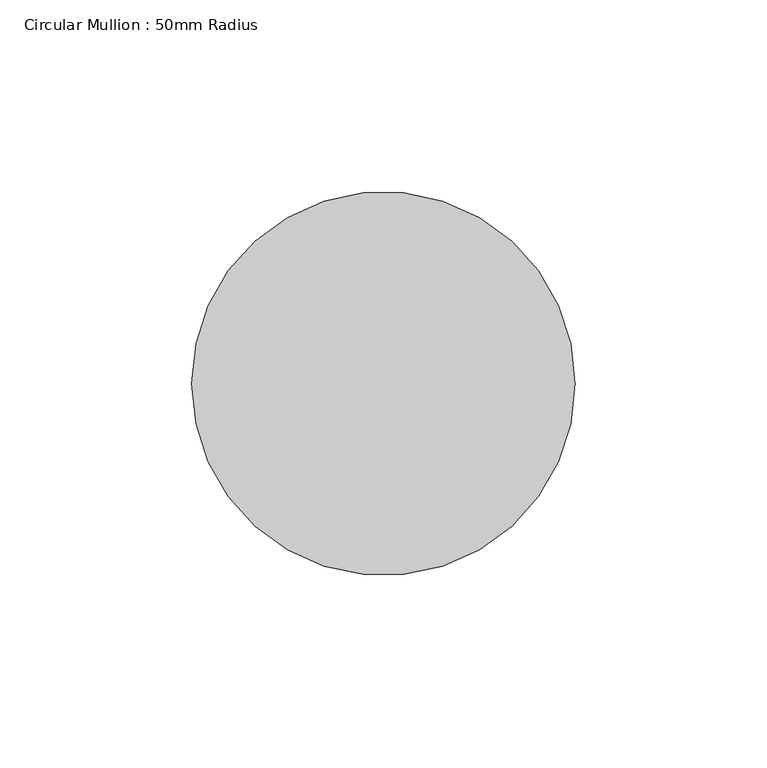
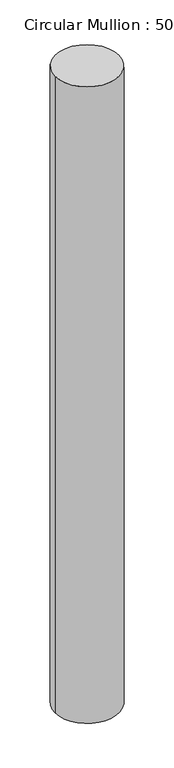
"""IFC4 building model written with IfcOpenShell, lengths in millimetres: member geometry, Circular Mullion : 50mm Radius."""

from ifc_helpers import new_model, si_unit, point, frame, origin, origin_2d, place, context, project, spatial, circle_curve, trimmed, segment, composite_curve, outline, extrude, source, transform, mapped, element, save


def circular_mullion_50mm_radius_49e016c5(model_context):
    return source(origin(), model_context, "Body", "SweptSolid", [
        extrude(outline(composite_curve([segment(trimmed(circle_curve(origin_2d(), 50.0), [point((50.0, 0.0))], [point((-50.0, 0.0))], False, "CARTESIAN"), True, "CONTINUOUS"), segment(trimmed(circle_curve(origin_2d(), 50.0), [point((-50.0, 0.0))], [point((50.0, 0.0))], False, "CARTESIAN"), True, "CONTINUOUS")], self_intersect=False)), frame((0.0, 0.0, -1053.810783), z_axis=(0.0, 0.0, 1.0), x_axis=(1.0, 0.0, 0.0)), (0.0, 0.0, 1.0), 1053.810783),
    ])


if __name__ == "__main__":
    model = new_model("IFC4")
    model_context = context("Model", 3, world=origin())
    ifc_project = project(units=[si_unit("LENGTHUNIT", "METRE", prefix="MILLI")], contexts=[model_context])
    site = spatial("IfcSite", under=ifc_project)
    building = spatial("IfcBuilding", under=site)
    placement = place(None, origin())
    circular_mullion_50mm_radius_shape = circular_mullion_50mm_radius_49e016c5(model_context)
    element("IfcMember", 1, ObjectType="Circular Mullion : 50mm Radius", at=placement, inside=building, context=model_context, shape_type="MappedRepresentation", body=[
        mapped(circular_mullion_50mm_radius_shape, transform((0.0, 0.0, 0.0), x_axis=(1.0, 0.0, 0.0), y_axis=(0.0, 1.0, 0.0), z_axis=(0.0, 0.0, 1.0))),
    ])
    save(model, "model.ifc")

# Revit data of these elements
# Type "Circular Mullion : 50mm Radius"
#   built-in parameter 1007350 = 0.164042 (stored number, unit not read)
# Element 1 (IfcMember, "Circular Mullion : 50mm Radius")
#   Materials on its faces: "Aluminium"
# Materials
#   "Aluminium": class "Metal", colour RGB 247 247 247, transparency 0, Description = "Aluminium 6061", Cost = 0
